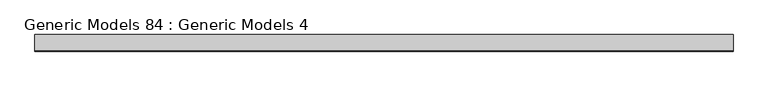
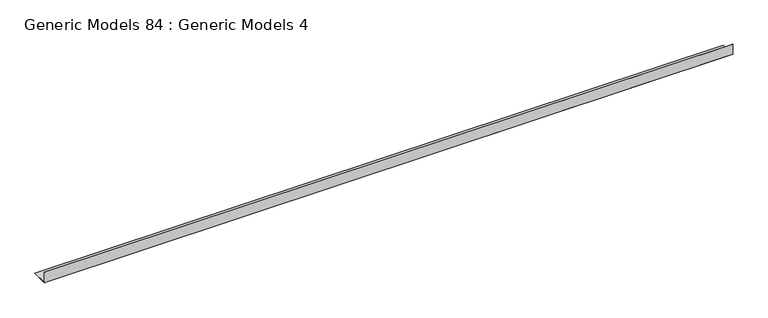
"""IFC4 building model written with IfcOpenShell, lengths in millimetres: proxy geometry, Generic Models 84 : Generic Models 4."""

from ifc_helpers import new_model, si_unit, frame, origin, place, context, project, spatial, polyline, outline, extrude, source, transform, mapped, element, save


def generic_models_84_generic_models_4_9c83ccc1(model_context):
    return source(origin(), model_context, "Body", "SweptSolid", [
        extrude(outline(polyline([(-6894.9800508, 126907.0294163), (-6748.0388625, 126903.9681416), (-6748.0553953, 126903.1745638), (-6895.7738008, 126906.2520306), (-6895.7738008, 127002.789691), (-6894.9800508, 127002.789691), (-6894.9800508, 126907.0294163)])), frame((2196.9263704, 0.0, 0.0), z_axis=(1.0, 0.0, 0.0), x_axis=(0.0, 1.0, 0.0)), (0.0, 0.0, 1.0), 6212.156498),
    ])


if __name__ == "__main__":
    model = new_model("IFC4")
    model_context = context("Model", 3, world=origin())
    ifc_project = project(units=[si_unit("LENGTHUNIT", "METRE", prefix="MILLI")], contexts=[model_context])
    site = spatial("IfcSite", under=ifc_project)
    building = spatial("IfcBuilding", under=site)
    placement = place(None, origin())
    generic_models_84_generic_models_4_shape = generic_models_84_generic_models_4_9c83ccc1(model_context)
    element("IfcBuildingElementProxy", 1, Name="Generic Models 84 : Generic Models 4", ObjectType="Generic Models 84 : Generic Models 4", at=placement, inside=building, context=model_context, shape_type="MappedRepresentation", body=[
        mapped(generic_models_84_generic_models_4_shape, transform((0.0, 0.0, 0.0), x_axis=(1.0, 0.0, 0.0), y_axis=(0.0, 1.0, 0.0), z_axis=(0.0, 0.0, 1.0))),
    ])
    save(model, "model.ifc")

# Revit data of these elements
# Element 1 (IfcBuildingElementProxy, "Generic Models 84 : Generic Models 4")
#   Materials on its faces: "_16 GA. COPPER \"L\" FLASHING - (6\" HORZ. LEG - 4\" VERT. LEG)"
# Materials
#   "_16 GA. COPPER \"L\" FLASHING - (6\" HORZ. LEG - 4\" VERT. LEG)": class "Generic", colour RGB 156 184 169, transparency 0, Cost = 0
